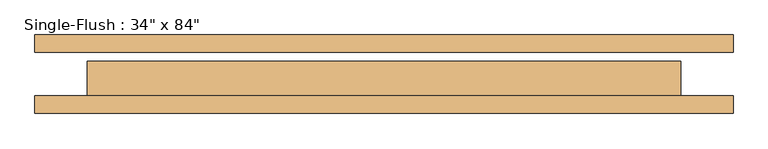
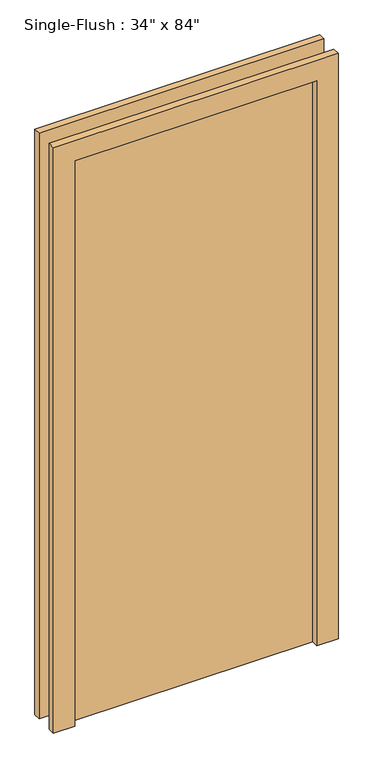
"""IFC4 building model written with IfcOpenShell, lengths in millimetres: door geometry."""

from ifc_helpers import new_model, si_unit, frame, origin, origin_with_axes, place, context, project, spatial, polyline, outline, extrude, source, transform, mapped, element, save


def door_21dfbfa2(model_context):
    return source(origin(), model_context, "Body", "SweptSolid", [
        extrude(outline(polyline([(2209.8, -508.0), (0.0, -508.0), (0.0, -431.8), (2133.6, -431.8), (2133.6, 431.8), (0.0, 431.8), (0.0, 508.0), (2209.8, 508.0), (2209.8, -508.0)])), frame((0.0, -57.15, 0.0), z_axis=(0.0, 1.0, 0.0), x_axis=(0.0, 0.0, 1.0)), (0.0, 0.0, 1.0), 25.4),
        extrude(outline(polyline([(2209.8, 508.0), (2209.8, -508.0), (0.0, -508.0), (0.0, -431.8), (2133.6, -431.8), (2133.6, 431.8), (0.0, 431.8), (0.0, 508.0), (2209.8, 508.0)])), frame((0.0, 31.75, 0.0), z_axis=(0.0, 1.0, 0.0), x_axis=(0.0, 0.0, 1.0)), (0.0, 0.0, 1.0), 25.4),
        extrude(outline(polyline([(431.8, 19.05), (431.8, -31.75), (-431.8, -31.75), (-431.8, 19.05), (431.8, 19.05)])), origin_with_axes(), (0.0, 0.0, 1.0), 2133.6),
    ])


if __name__ == "__main__":
    model = new_model("IFC4")
    model_context = context("Model", 3, world=origin())
    ifc_project = project(units=[si_unit("LENGTHUNIT", "METRE", prefix="MILLI")], contexts=[model_context])
    site = spatial("IfcSite", under=ifc_project)
    building = spatial("IfcBuilding", under=site)
    placement = place(None, origin())
    door_shape = door_21dfbfa2(model_context)
    element("IfcDoor", 1, ObjectType="Single-Flush : 34\" x 84\"", at=placement, inside=building, context=model_context, shape_type="MappedRepresentation", body=[
        mapped(door_shape, transform((0.0, 0.0, 0.0), x_axis=(1.0, 0.0, 0.0), y_axis=(0.0, 1.0, 0.0), z_axis=(0.0, 0.0, 1.0))),
    ])
    save(model, "model.ifc")

# Revit data of these elements
# Type "Single-Flush : 34\" x 84\""
#   Type Mark = "2"
#   Construction Type Id = "MDOOR"
#   Assembly Code = "C1020"
#   Analytic Construction = "Metal"
#   Thickness = 0' - 2"
#   Heat Transfer Coefficient (U) = 0.651978 BTU/(h·ft²·°F)
#   Height = 7' - 0"
#   Trim Projection Ext = 0' - 1"
#   Trim Projection Int = 0' - 1"
#   Trim Width = 0' - 3"
#   Width = 2' - 10"
#   Define Thermal Properties by = 1
#   Define Thermal Properties by = 1
#   Door Material = Door - Panel
#   Frame Material = Door - Frame
#   Visual Light Transmittance = 0
#   Solar Heat Gain Coefficient = 0
#   Function = (empty or 0)
#   Wall Closure = (empty or 0)
# Element 1 (IfcDoor, "Single-Flush : 34\" x 84\"")
#   Materials on its faces: "Door - Frame", "Door - Panel"
# Materials
#   "Door - Panel": class "Wood", colour RGB 210 159 95, transparency 0, Cost = 0
#   "Door - Frame": class "Miscellaneous", colour RGB 118 70 51, transparency 0, Cost = 0
